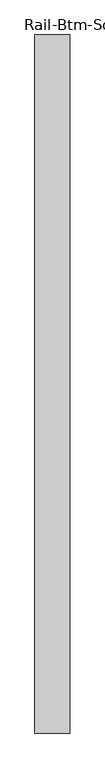
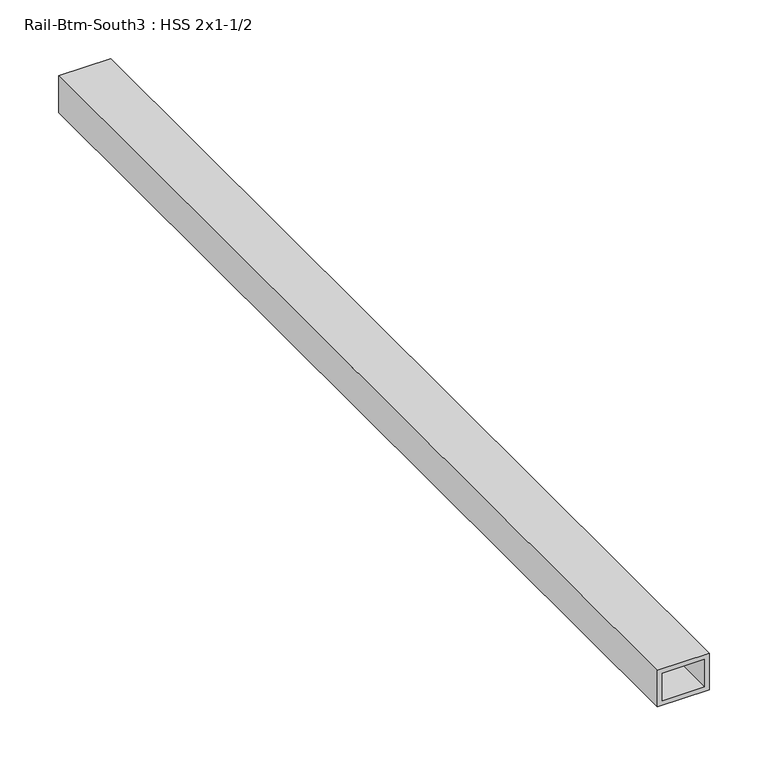
"""IFC4 building model written with IfcOpenShell, lengths in millimetres: proxy geometry, Rail-Btm-South3 : HSS 2x1-1/2."""

import ifcopenshell
import ifcopenshell.guid

model = None  # the IFC model being written
_history = None  # IfcOwnerHistory: only IFC2X3 demands one
_inside = {}  # id of a spatial element -> (the spatial element, [elements in it])
_under = {}  # id of a project, library or spatial element -> (it, [spatial elements below it])
_declared = {}  # id of a project -> (the project, [libraries it declares])
_typed = {}  # id of a type object -> (the type object, [elements of that type])
_made_of = {}  # id of a material, layer set ... -> (it, [elements and type objects made of it])


def new_model(schema):
    """Start an empty IFC model of exactly this schema.

    Asked for "IFC4X3", IfcOpenShell would pick the latest addendum, in which some entities
    have other attributes; the version numbers below select the first issue.
    IFC2X3 requires an IfcOwnerHistory on every rooted entity: one is made here for all.
    """
    global model, _history
    if schema == "IFC4X3":
        model = ifcopenshell.file(schema_version=(4, 3, 0, 0))
    else:
        model = ifcopenshell.file(schema=schema)
    _inside.clear()
    _under.clear()
    _declared.clear()
    _typed.clear()
    _made_of.clear()
    _history = None
    if model.schema == "IFC2X3":
        org = make("IfcOrganization", Name="unknown")
        user = make(
            "IfcPersonAndOrganization",
            ThePerson=make("IfcPerson", FamilyName="unknown"),
            TheOrganization=org,
        )
        app = make(
            "IfcApplication",
            ApplicationDeveloper=org,
            Version="unknown",
            ApplicationFullName="unknown",
            ApplicationIdentifier="unknown",
        )
        _history = make(
            "IfcOwnerHistory",
            OwningUser=user,
            OwningApplication=app,
            ChangeAction="ADDED",
            CreationDate=0,
        )
    return model


def make(cls, **values):
    """One entity of the class cls with the attributes given. An attribute that is None is left unset."""
    return model.create_entity(
        cls, **{name: value for name, value in values.items() if value is not None}
    )


def rooted(cls, **values):
    """An entity with a GlobalId (a new one), such as an element, a storey or a relation."""
    return make(cls, GlobalId=ifcopenshell.guid.new(), OwnerHistory=_history, **values)


def si_unit(unit_type, name, prefix=None):
    """IfcSIUnit, for example si_unit("LENGTHUNIT", "METRE", prefix="MILLI")."""
    return make("IfcSIUnit", UnitType=unit_type, Prefix=prefix, Name=name)


def assignment(units):
    """IfcUnitAssignment: the units of a project."""
    return None if units is None else make("IfcUnitAssignment", Units=units)


def point(xyz):
    """IfcCartesianPoint."""
    return None if xyz is None else make("IfcCartesianPoint", Coordinates=xyz)


def direction(xyz):
    """IfcDirection."""
    return None if xyz is None else make("IfcDirection", DirectionRatios=xyz)


def frame(location, z_axis=None, x_axis=None):
    """IfcAxis2Placement3D, a coordinate frame: its origin and axes. An axis left out is left unset."""
    return make(
        "IfcAxis2Placement3D",
        Location=point(location),
        Axis=direction(z_axis),
        RefDirection=direction(x_axis),
    )


def origin():
    """The frame at (0, 0, 0) with its axes left unset."""
    return frame((0.0, 0.0, 0.0))


def place(relative_to, where):
    """IfcLocalPlacement: puts the frame where relative to a parent placement (None: the world)."""
    return make(
        "IfcLocalPlacement", PlacementRelTo=relative_to, RelativePlacement=where
    )


def context(
    kind, dimensions, precision=None, world=None, true_north=None, identifier=None
):
    """IfcGeometricRepresentationContext, for example the 3D "Model" context."""
    return make(
        "IfcGeometricRepresentationContext",
        ContextIdentifier=identifier,
        ContextType=kind,
        CoordinateSpaceDimension=dimensions,
        Precision=precision,
        WorldCoordinateSystem=world,
        TrueNorth=true_north,
    )


def project(units=None, contexts=None):
    """IfcProject with its units and contexts."""
    return rooted(
        "IfcProject",
        Name="project",
        RepresentationContexts=contexts,
        UnitsInContext=assignment(units),
    )


def spatial(cls, under=None, at=None, **own):
    """A site, building, storey or space (cls), placed at a placement, below another one or the project."""
    s = rooted(cls, ObjectPlacement=at, **own)
    if under is not None:
        _under.setdefault(under.id(), (under, []))[1].append(s)
    return s


def polyline(points):
    """IfcPolyline through the points."""
    return make("IfcPolyline", Points=[point(p) for p in points])


def outline(outer, holes=None, kind="AREA"):
    """IfcArbitraryClosedProfileDef: a profile drawn as a closed curve; with holes, ...WithVoids."""
    if holes is None:
        return make("IfcArbitraryClosedProfileDef", ProfileType=kind, OuterCurve=outer)
    return make(
        "IfcArbitraryProfileDefWithVoids",
        ProfileType=kind,
        OuterCurve=outer,
        InnerCurves=holes,
    )


def extrude(swept, where, along, depth):
    """IfcExtrudedAreaSolid: the profile swept, set in the frame where, extruded along a direction by depth."""
    return make(
        "IfcExtrudedAreaSolid",
        SweptArea=swept,
        Position=where,
        ExtrudedDirection=direction(along),
        Depth=depth,
    )


def shape(context_of_items, identifier, shape_type, items):
    """IfcShapeRepresentation: the items that make up one representation, for example the "Body"."""
    return make(
        "IfcShapeRepresentation",
        ContextOfItems=context_of_items,
        RepresentationIdentifier=identifier,
        RepresentationType=shape_type,
        Items=items,
    )


def source(mapping_origin, context_of_items, identifier, shape_type, items):
    """IfcRepresentationMap: a shape defined once, which mapped items show again and again."""
    return make(
        "IfcRepresentationMap",
        MappingOrigin=mapping_origin,
        MappedRepresentation=shape(context_of_items, identifier, shape_type, items),
    )


def transform(
    local_origin,
    x_axis=None,
    y_axis=None,
    z_axis=None,
    scale=None,
    scale2=None,
    scale3=None,
    uniform=True,
):
    """IfcCartesianTransformationOperator3D, or its non-uniform kind. x_axis, y_axis, z_axis: its Axis1, 2, 3."""
    if uniform:
        return make(
            "IfcCartesianTransformationOperator3D",
            Axis1=direction(x_axis),
            Axis2=direction(y_axis),
            LocalOrigin=point(local_origin),
            Scale=scale,
            Axis3=direction(z_axis),
        )
    return make(
        "IfcCartesianTransformationOperator3DnonUniform",
        Axis1=direction(x_axis),
        Axis2=direction(y_axis),
        LocalOrigin=point(local_origin),
        Scale=scale,
        Axis3=direction(z_axis),
        Scale2=scale2,
        Scale3=scale3,
    )


def mapped(mapping_source, mapping_target):
    """IfcMappedItem: shows the shape of a source again, moved by a transform."""
    return make(
        "IfcMappedItem", MappingSource=mapping_source, MappingTarget=mapping_target
    )


def made_of(thing, what):
    """Note that an element or type object is made of a material, layer set ...; save() writes the relation."""
    if what is not None:
        _made_of.setdefault(what.id(), (what, []))[1].append(thing)
    return thing


def element(
    cls,
    number,
    at=None,
    inside=None,
    cuts=None,
    type_object=None,
    material=None,
    context=None,
    identifier="Body",
    shape_type=None,
    held_by="IfcProductDefinitionShape",
    body=None,
    shapes=None,
    **own,
):
    """One element of the class cls, such as IfcWall. Its Tag is "e" and its number.

    at: its placement. inside: the storey or other place that contains it. cuts: it is an
    opening in that element (IfcRelVoidsElement). A single representation is given by context,
    identifier, shape_type and body (its items); several are given by shapes. held_by: the class
    of the entity that holds the representations. save() writes the other relations.
    """
    e = rooted(cls, Tag="e%d" % number, ObjectPlacement=at, **own)
    if body is not None:
        shapes = [shape(context, identifier, shape_type, body)]
    if shapes is not None:
        e.Representation = make(held_by, Representations=shapes)
    if inside is not None:
        _inside.setdefault(inside.id(), (inside, []))[1].append(e)
    if cuts is not None:
        rooted(
            "IfcRelVoidsElement", RelatingBuildingElement=cuts, RelatedOpeningElement=e
        )
    if type_object is not None:
        _typed.setdefault(type_object.id(), (type_object, []))[1].append(e)
    return made_of(e, material)


def aggregate(whole, parts):
    """IfcRelAggregates: a whole, such as a stair, and the parts it consists of."""
    return rooted("IfcRelAggregates", RelatingObject=whole, RelatedObjects=parts)


def save(model, path):
    """Write the relations noted so far, then the file.

    IfcRelAggregates (storeys below a building ...), IfcRelContainedInSpatialStructure (elements
    in a storey), IfcRelDefinesByType, IfcRelAssociatesMaterial and IfcRelDeclares: one each for
    every whole, place, type object, material and project.
    """
    for whole, parts in _under.values():
        aggregate(whole, parts)
    for where, things in _inside.values():
        rooted(
            "IfcRelContainedInSpatialStructure",
            RelatedElements=things,
            RelatingStructure=where,
        )
    for kind, things in _typed.values():
        rooted("IfcRelDefinesByType", RelatedObjects=things, RelatingType=kind)
    for what, things in _made_of.values():
        rooted("IfcRelAssociatesMaterial", RelatedObjects=things, RelatingMaterial=what)
    for by, libraries in _declared.values():
        rooted("IfcRelDeclares", RelatingContext=by, RelatedDefinitions=libraries)
    model.write(path)


def rail_btm_south3_hss_2x1_1_2_3e8d5585(model_context):
    return source(origin(), model_context, "Body", "SweptSolid", [
        extrude(outline(polyline([(50.8, 587416.6934739), (88.9, 587416.6934739), (88.9, 587365.8934739), (50.8, 587365.8934739), (50.8, 587416.6934739)]), holes=[polyline([(84.1375, 587411.9309739), (55.5625, 587411.9309739), (55.5625, 587370.6559739), (84.1375, 587370.6559739), (84.1375, 587411.9309739)])]), frame((0.0, -536263.6038841, 0.0), z_axis=(0.0, 1.0, 0.0), x_axis=(0.0, 0.0, 1.0)), (0.0, 0.0, 1.0), 1017.5875),
    ])


if __name__ == "__main__":
    model = new_model("IFC4")
    model_context = context("Model", 3, world=origin())
    ifc_project = project(units=[si_unit("LENGTHUNIT", "METRE", prefix="MILLI")], contexts=[model_context])
    site = spatial("IfcSite", under=ifc_project)
    building = spatial("IfcBuilding", under=site)
    placement = place(None, origin())
    rail_btm_south3_hss_2x1_1_2_shape = rail_btm_south3_hss_2x1_1_2_3e8d5585(model_context)
    element("IfcBuildingElementProxy", 1, Name="Rail-Btm-South3 : HSS 2x1-1/2", ObjectType="Rail-Btm-South3 : HSS 2x1-1/2", at=placement, inside=building, context=model_context, shape_type="MappedRepresentation", body=[
        mapped(rail_btm_south3_hss_2x1_1_2_shape, transform((0.0, 0.0, 0.0), x_axis=(1.0, 0.0, 0.0), y_axis=(0.0, 1.0, 0.0), z_axis=(0.0, 0.0, 1.0))),
    ])
    save(model, "model.ifc")

# Revit data of these elements
# Element 1 (IfcBuildingElementProxy, "Rail-Btm-South3 : HSS 2x1-1/2")
#   Materials on its faces: "1-1/2\"X2\" GALV. STL HSS TUBING"
# Materials
#   "1-1/2\"X2\" GALV. STL HSS TUBING": class "Generic", colour RGB 211 211 207, transparency 0, Cost = 0
